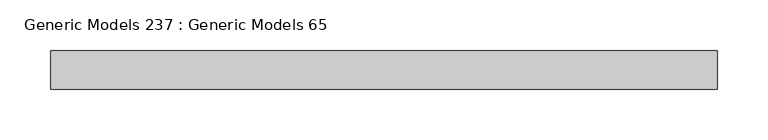
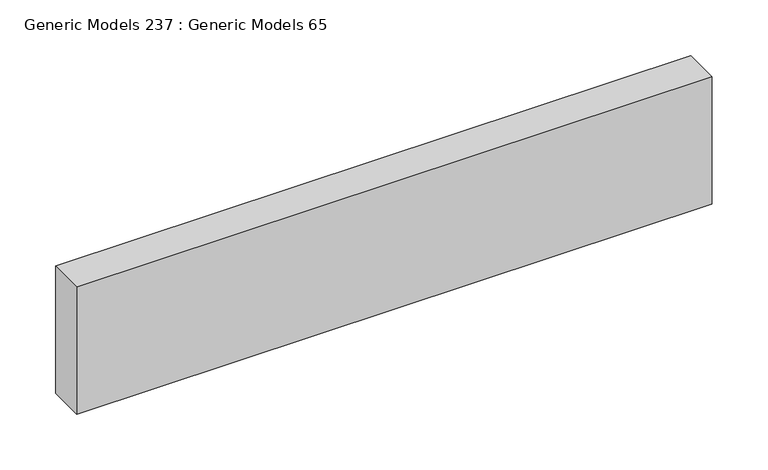
"""IFC4 building model written with IfcOpenShell, lengths in millimetres: proxy geometry, Generic Models 237 : Generic Models 65."""

import ifcopenshell
import ifcopenshell.guid

model = None  # the IFC model being written
_history = None  # IfcOwnerHistory: only IFC2X3 demands one
_inside = {}  # id of a spatial element -> (the spatial element, [elements in it])
_under = {}  # id of a project, library or spatial element -> (it, [spatial elements below it])
_declared = {}  # id of a project -> (the project, [libraries it declares])
_typed = {}  # id of a type object -> (the type object, [elements of that type])
_made_of = {}  # id of a material, layer set ... -> (it, [elements and type objects made of it])


def new_model(schema):
    """Start an empty IFC model of exactly this schema.

    Asked for "IFC4X3", IfcOpenShell would pick the latest addendum, in which some entities
    have other attributes; the version numbers below select the first issue.
    IFC2X3 requires an IfcOwnerHistory on every rooted entity: one is made here for all.
    """
    global model, _history
    if schema == "IFC4X3":
        model = ifcopenshell.file(schema_version=(4, 3, 0, 0))
    else:
        model = ifcopenshell.file(schema=schema)
    _inside.clear()
    _under.clear()
    _declared.clear()
    _typed.clear()
    _made_of.clear()
    _history = None
    if model.schema == "IFC2X3":
        org = make("IfcOrganization", Name="unknown")
        user = make(
            "IfcPersonAndOrganization",
            ThePerson=make("IfcPerson", FamilyName="unknown"),
            TheOrganization=org,
        )
        app = make(
            "IfcApplication",
            ApplicationDeveloper=org,
            Version="unknown",
            ApplicationFullName="unknown",
            ApplicationIdentifier="unknown",
        )
        _history = make(
            "IfcOwnerHistory",
            OwningUser=user,
            OwningApplication=app,
            ChangeAction="ADDED",
            CreationDate=0,
        )
    return model


def make(cls, **values):
    """One entity of the class cls with the attributes given. An attribute that is None is left unset."""
    return model.create_entity(
        cls, **{name: value for name, value in values.items() if value is not None}
    )


def rooted(cls, **values):
    """An entity with a GlobalId (a new one), such as an element, a storey or a relation."""
    return make(cls, GlobalId=ifcopenshell.guid.new(), OwnerHistory=_history, **values)


def si_unit(unit_type, name, prefix=None):
    """IfcSIUnit, for example si_unit("LENGTHUNIT", "METRE", prefix="MILLI")."""
    return make("IfcSIUnit", UnitType=unit_type, Prefix=prefix, Name=name)


def assignment(units):
    """IfcUnitAssignment: the units of a project."""
    return None if units is None else make("IfcUnitAssignment", Units=units)


def point(xyz):
    """IfcCartesianPoint."""
    return None if xyz is None else make("IfcCartesianPoint", Coordinates=xyz)


def direction(xyz):
    """IfcDirection."""
    return None if xyz is None else make("IfcDirection", DirectionRatios=xyz)


def frame(location, z_axis=None, x_axis=None):
    """IfcAxis2Placement3D, a coordinate frame: its origin and axes. An axis left out is left unset."""
    return make(
        "IfcAxis2Placement3D",
        Location=point(location),
        Axis=direction(z_axis),
        RefDirection=direction(x_axis),
    )


def origin():
    """The frame at (0, 0, 0) with its axes left unset."""
    return frame((0.0, 0.0, 0.0))


def place(relative_to, where):
    """IfcLocalPlacement: puts the frame where relative to a parent placement (None: the world)."""
    return make(
        "IfcLocalPlacement", PlacementRelTo=relative_to, RelativePlacement=where
    )


def context(
    kind, dimensions, precision=None, world=None, true_north=None, identifier=None
):
    """IfcGeometricRepresentationContext, for example the 3D "Model" context."""
    return make(
        "IfcGeometricRepresentationContext",
        ContextIdentifier=identifier,
        ContextType=kind,
        CoordinateSpaceDimension=dimensions,
        Precision=precision,
        WorldCoordinateSystem=world,
        TrueNorth=true_north,
    )


def project(units=None, contexts=None):
    """IfcProject with its units and contexts."""
    return rooted(
        "IfcProject",
        Name="project",
        RepresentationContexts=contexts,
        UnitsInContext=assignment(units),
    )


def spatial(cls, under=None, at=None, **own):
    """A site, building, storey or space (cls), placed at a placement, below another one or the project."""
    s = rooted(cls, ObjectPlacement=at, **own)
    if under is not None:
        _under.setdefault(under.id(), (under, []))[1].append(s)
    return s


def polyline(points):
    """IfcPolyline through the points."""
    return make("IfcPolyline", Points=[point(p) for p in points])


def outline(outer, holes=None, kind="AREA"):
    """IfcArbitraryClosedProfileDef: a profile drawn as a closed curve; with holes, ...WithVoids."""
    if holes is None:
        return make("IfcArbitraryClosedProfileDef", ProfileType=kind, OuterCurve=outer)
    return make(
        "IfcArbitraryProfileDefWithVoids",
        ProfileType=kind,
        OuterCurve=outer,
        InnerCurves=holes,
    )


def extrude(swept, where, along, depth):
    """IfcExtrudedAreaSolid: the profile swept, set in the frame where, extruded along a direction by depth."""
    return make(
        "IfcExtrudedAreaSolid",
        SweptArea=swept,
        Position=where,
        ExtrudedDirection=direction(along),
        Depth=depth,
    )


def shape(context_of_items, identifier, shape_type, items):
    """IfcShapeRepresentation: the items that make up one representation, for example the "Body"."""
    return make(
        "IfcShapeRepresentation",
        ContextOfItems=context_of_items,
        RepresentationIdentifier=identifier,
        RepresentationType=shape_type,
        Items=items,
    )


def source(mapping_origin, context_of_items, identifier, shape_type, items):
    """IfcRepresentationMap: a shape defined once, which mapped items show again and again."""
    return make(
        "IfcRepresentationMap",
        MappingOrigin=mapping_origin,
        MappedRepresentation=shape(context_of_items, identifier, shape_type, items),
    )


def transform(
    local_origin,
    x_axis=None,
    y_axis=None,
    z_axis=None,
    scale=None,
    scale2=None,
    scale3=None,
    uniform=True,
):
    """IfcCartesianTransformationOperator3D, or its non-uniform kind. x_axis, y_axis, z_axis: its Axis1, 2, 3."""
    if uniform:
        return make(
            "IfcCartesianTransformationOperator3D",
            Axis1=direction(x_axis),
            Axis2=direction(y_axis),
            LocalOrigin=point(local_origin),
            Scale=scale,
            Axis3=direction(z_axis),
        )
    return make(
        "IfcCartesianTransformationOperator3DnonUniform",
        Axis1=direction(x_axis),
        Axis2=direction(y_axis),
        LocalOrigin=point(local_origin),
        Scale=scale,
        Axis3=direction(z_axis),
        Scale2=scale2,
        Scale3=scale3,
    )


def mapped(mapping_source, mapping_target):
    """IfcMappedItem: shows the shape of a source again, moved by a transform."""
    return make(
        "IfcMappedItem", MappingSource=mapping_source, MappingTarget=mapping_target
    )


def made_of(thing, what):
    """Note that an element or type object is made of a material, layer set ...; save() writes the relation."""
    if what is not None:
        _made_of.setdefault(what.id(), (what, []))[1].append(thing)
    return thing


def element(
    cls,
    number,
    at=None,
    inside=None,
    cuts=None,
    type_object=None,
    material=None,
    context=None,
    identifier="Body",
    shape_type=None,
    held_by="IfcProductDefinitionShape",
    body=None,
    shapes=None,
    **own,
):
    """One element of the class cls, such as IfcWall. Its Tag is "e" and its number.

    at: its placement. inside: the storey or other place that contains it. cuts: it is an
    opening in that element (IfcRelVoidsElement). A single representation is given by context,
    identifier, shape_type and body (its items); several are given by shapes. held_by: the class
    of the entity that holds the representations. save() writes the other relations.
    """
    e = rooted(cls, Tag="e%d" % number, ObjectPlacement=at, **own)
    if body is not None:
        shapes = [shape(context, identifier, shape_type, body)]
    if shapes is not None:
        e.Representation = make(held_by, Representations=shapes)
    if inside is not None:
        _inside.setdefault(inside.id(), (inside, []))[1].append(e)
    if cuts is not None:
        rooted(
            "IfcRelVoidsElement", RelatingBuildingElement=cuts, RelatedOpeningElement=e
        )
    if type_object is not None:
        _typed.setdefault(type_object.id(), (type_object, []))[1].append(e)
    return made_of(e, material)


def aggregate(whole, parts):
    """IfcRelAggregates: a whole, such as a stair, and the parts it consists of."""
    return rooted("IfcRelAggregates", RelatingObject=whole, RelatedObjects=parts)


def save(model, path):
    """Write the relations noted so far, then the file.

    IfcRelAggregates (storeys below a building ...), IfcRelContainedInSpatialStructure (elements
    in a storey), IfcRelDefinesByType, IfcRelAssociatesMaterial and IfcRelDeclares: one each for
    every whole, place, type object, material and project.
    """
    for whole, parts in _under.values():
        aggregate(whole, parts)
    for where, things in _inside.values():
        rooted(
            "IfcRelContainedInSpatialStructure",
            RelatedElements=things,
            RelatingStructure=where,
        )
    for kind, things in _typed.values():
        rooted("IfcRelDefinesByType", RelatedObjects=things, RelatingType=kind)
    for what, things in _made_of.values():
        rooted("IfcRelAssociatesMaterial", RelatedObjects=things, RelatingMaterial=what)
    for by, libraries in _declared.values():
        rooted("IfcRelDeclares", RelatingContext=by, RelatedDefinitions=libraries)
    model.write(path)


def generic_models_237_generic_models_65_1df05f16(model_context):
    return source(origin(), model_context, "Body", "SweptSolid", [
        extrude(outline(polyline([(48469.55, 592.1375), (48469.55, 630.2375), (49128.3625, 630.2375), (49128.3625, 592.1375), (48469.55, 592.1375)])), frame((0.0, 0.0, 5507.83125), z_axis=(0.0, 0.0, 1.0), x_axis=(1.0, 0.0, 0.0)), (0.0, 0.0, 1.0), 139.7),
    ])


if __name__ == "__main__":
    model = new_model("IFC4")
    model_context = context("Model", 3, world=origin())
    ifc_project = project(units=[si_unit("LENGTHUNIT", "METRE", prefix="MILLI")], contexts=[model_context])
    site = spatial("IfcSite", under=ifc_project)
    building = spatial("IfcBuilding", under=site)
    placement = place(None, origin())
    generic_models_237_generic_models_65_shape = generic_models_237_generic_models_65_1df05f16(model_context)
    element("IfcBuildingElementProxy", 1, Name="Generic Models 237 : Generic Models 65", ObjectType="Generic Models 237 : Generic Models 65", at=placement, inside=building, context=model_context, shape_type="MappedRepresentation", body=[
        mapped(generic_models_237_generic_models_65_shape, transform((0.0, 0.0, 0.0), x_axis=(1.0, 0.0, 0.0), y_axis=(0.0, 1.0, 0.0), z_axis=(0.0, 0.0, 1.0))),
    ])
    save(model, "model.ifc")

# Revit data of these elements
# Element 1 (IfcBuildingElementProxy, "Generic Models 237 : Generic Models 65")
#   Materials on its faces: "WOOD JOIST AS SPECIFIED"
# Materials
#   "WOOD JOIST AS SPECIFIED": class "Wood", colour RGB 234 198 147, transparency 0, Description = "Pinus Echinata", Cost = 0
